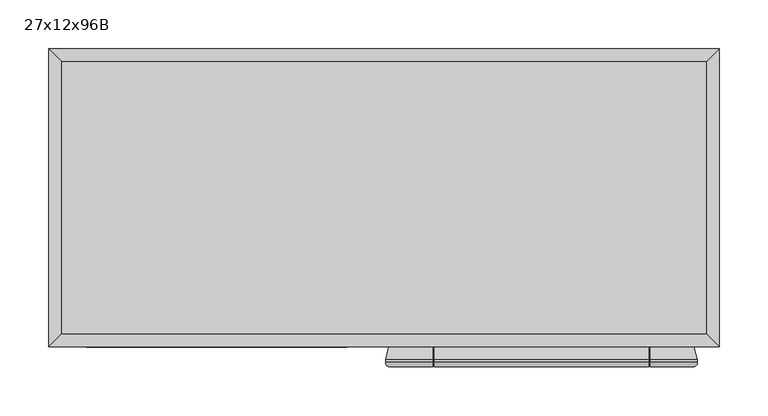
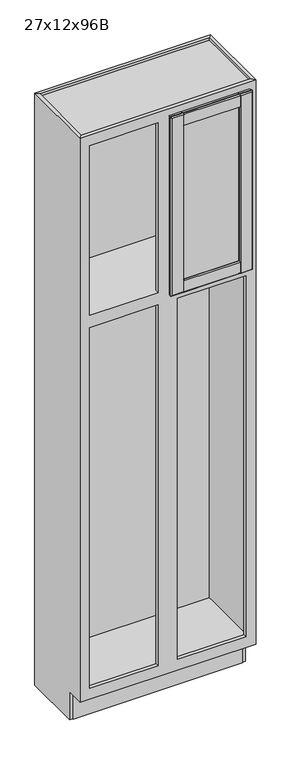
"""IFC4 building model written with IfcOpenShell, lengths in millimetres: furniture geometry, Cabinet-Tall-Merillat-Utility_Double-Marlin : 27x12x96B."""

from ifc_helpers import new_model, si_unit, frame, origin, origin_with_axes, place, context, project, spatial, polyline, circle_curve, ellipse_curve, outline, extrude, faceted_brep, source, transform, mapped, element, save
from ifc_brep_helpers import plane_surface, cylinder_surface, advanced_brep


def furniture_27x12x96b_0ef1cbea(model_context):
    return source(origin(), model_context, "Body", "SolidModel", [
        advanced_brep(
        [(314.6646592, -320.6496, 2413.0), (311.5681667, -325.12, 2409.9035075), (311.5681667, -325.12, 1679.4964925), (314.6646592, -320.6496, 1676.4), (314.6646592, -317.881, 1676.4), (314.6646592, -317.881, 2413.0), (311.1594592, -304.8, 1679.9052), (311.1594592, -304.8, 2409.4948), (266.4634964, -304.8, 2364.7988372), (266.4634964, -304.8, 1724.6011628), (266.0933647, -305.59375, 1724.9712945), (264.0122057, -310.05681, 1727.0524535), (264.0122057, -310.05681, 2362.3475465), (266.0933647, -305.59375, 2364.4287055), (265.4119751, -312.2969093, 1725.652684), (265.4119751, -312.2969093, 2363.747316), (279.7396592, -312.547, 1711.325), (279.7396592, -312.547, 2378.075), (279.7396592, -317.373, 1711.325), (279.7396592, -317.373, 2378.075), (265.4119751, -317.6230907, 1725.652684), (265.4119751, -317.6230907, 2363.747316), (264.0122057, -319.86319, 1727.0524535), (264.0122057, -319.86319, 2362.3475465), (266.0933647, -324.32625, 1724.9712945), (266.460629, -325.1138508, 1724.6040302), (266.4634964, -325.12, 2364.7988372), (266.0933647, -324.32625, 2364.4287055), (266.460629, -325.12, 1679.4964925), (266.460629, -320.6496, 1676.4), (-1.3263483, -325.12, 1679.4964925), (-4.4228408, -320.6496, 1676.4), (43.7413778, -320.6496, 1676.4), (43.7413778, -325.12, 1679.4964925), (264.873129, -320.6496, 1676.4), (264.873129, -325.12, 1679.4964925), (45.3288778, -325.12, 1679.4964925), (45.3288778, -320.6496, 1676.4), (266.460629, -317.881, 1676.4), (-4.4228408, -317.881, 1676.4), (43.7413778, -317.881, 1676.4), (264.873129, -317.881, 1676.4), (45.3288778, -317.881, 1676.4), (266.460629, -304.8, 1679.9052), (-0.9176408, -304.8, 1679.9052), (43.7413778, -304.8, 1679.9052), (264.873129, -304.8, 1679.9052), (45.3288778, -304.8, 1679.9052), (46.2296127, -310.05681, 1727.0524535), (264.873129, -305.59375, 1724.9712945), (264.873129, -304.8, 1724.6011628), (45.3288778, -304.8, 1724.6011628), (45.3288778, -305.59375, 1724.9712945), (44.1484536, -305.59375, 1724.9712945), (44.8298432, -312.2969093, 1725.652684), (30.5021592, -312.547, 1711.325), (30.5021592, -317.373, 1711.325), (44.8298432, -317.6230907, 1725.652684), (46.2296127, -319.86319, 1727.0524535), (44.1484536, -324.32625, 1724.9712945), (45.3288778, -324.32625, 1724.9712945), (45.3288778, -325.12, 1724.6011628), (264.873129, -325.12, 1724.6011628), (264.873129, -324.32625, 1724.9712945), (-1.3263483, -325.12, 2409.9035075), (-4.4228408, -320.6496, 2413.0), (-4.4228408, -317.881, 2413.0), (-0.9176408, -304.8, 2409.4948), (43.7783219, -304.8, 1724.6011628), (43.7783219, -304.8, 2364.7988372), (44.1484536, -305.59375, 2364.4287055), (46.2296127, -310.05681, 2362.3475465), (44.8298432, -312.2969093, 2363.747316), (30.5021592, -312.547, 2378.075), (30.5021592, -317.373, 2378.075), (44.8298432, -317.6230907, 2363.747316), (46.2296127, -319.86319, 2362.3475465), (44.1484536, -324.32625, 2364.4287055), (43.7783219, -325.12, 2364.7988372), (43.7783219, -325.12, 1724.6011628), (43.7413778, -325.12, 2409.9035075), (43.7413778, -320.6496, 2413.0), (266.460629, -320.6496, 2413.0), (266.460629, -325.12, 2409.9035075), (45.3288778, -320.6496, 2413.0), (45.3288778, -325.12, 2409.9035075), (264.873129, -325.12, 2409.9035075), (264.873129, -320.6496, 2413.0), (43.7413778, -317.881, 2413.0), (266.460629, -317.881, 2413.0), (45.3288778, -317.881, 2413.0), (264.873129, -317.881, 2413.0), (43.7413778, -304.8, 2409.4948), (266.460629, -304.8, 2409.4948), (45.3288778, -304.8, 2409.4948), (264.873129, -304.8, 2409.4948), (45.3288778, -304.8, 2364.7988372), (264.873129, -304.8, 2364.7988372), (45.3288778, -305.59375, 2364.4287055), (264.873129, -305.59375, 2364.4287055), (264.873129, -324.32625, 2364.4287055), (264.873129, -325.12, 2364.7988372), (45.3288778, -325.12, 2364.7988372), (45.3288778, -324.32625, 2364.4287055), (45.3288778, -305.59375, 2408.8857412), (45.3288778, -317.9855037, 2412.20625), (45.3288778, -320.6496, 2412.20625), (45.3288778, -324.32625, 2409.7526052), (43.7413778, -324.32625, 2364.4287055), (43.7413778, -324.32625, 2409.7526052), (43.7413778, -320.6496, 2412.20625), (43.7413778, -317.9855037, 2412.20625), (43.7413778, -305.59375, 2408.8857412), (43.7413778, -305.59375, 2364.4287055), (266.460629, -305.59375, 2364.4287055), (266.460629, -305.59375, 2408.8857412), (266.460629, -317.9855037, 2412.20625), (266.460629, -320.6496, 2412.20625), (266.460629, -324.32625, 2409.7526052), (266.460629, -324.32625, 2364.4287055), (264.873129, -324.32625, 2409.7526052), (264.873129, -320.6496, 2412.20625), (264.873129, -317.9855037, 2412.20625), (264.873129, -305.59375, 2408.8857412), (266.460629, -324.32625, 1724.9712945), (266.460629, -324.32625, 1679.6473948), (266.460629, -320.6496, 1677.19375), (266.460629, -317.9855037, 1677.19375), (266.460629, -305.59375, 1680.5142588), (266.460629, -305.59375, 1724.9712945), (264.873129, -305.59375, 1680.5142588), (264.873129, -317.9855037, 1677.19375), (264.873129, -320.6496, 1677.19375), (264.873129, -324.32625, 1679.6473948), (45.3288778, -324.32625, 1679.6473948), (45.3288778, -320.6496, 1677.19375), (45.3288778, -317.9855037, 1677.19375), (45.3288778, -305.59375, 1680.5142588), (43.7413778, -324.32625, 1724.9712945), (43.7413778, -305.59375, 1724.9712945), (43.7413778, -305.59375, 1680.5142588), (43.7413778, -317.9855037, 1677.19375), (43.7413778, -320.6496, 1677.19375), (43.7413778, -324.32625, 1679.6473948)],
        [
            (0, 1, ellipse_curve(frame((309.8894592, -320.6496, 2408.2248), z_axis=(0.7071067811865475, 0.0, -0.7071067811865475), x_axis=(0.7071067811865474, 0.0, 0.7071067811865476)), 6.7531526, 4.7752)),
            (1, 2),
            (2, 3, ellipse_curve(frame((309.8894592, -320.6496, 1681.1752), z_axis=(0.7071067811865475, 0.0, 0.7071067811865475), x_axis=(-0.7071067811865474, 0.0, 0.7071067811865476)), 6.7531526, 4.7752)),
            (3, 0),
            (3, 4),
            (4, 5),
            (5, 0),
            (4, 6),
            (6, 7),
            (7, 5),
            (8, 9),
            (9, 10),
            (10, 11),
            (11, 12),
            (12, 13),
            (13, 8),
            (11, 14, ellipse_curve(frame((265.4394592, -310.7223492, 1725.6252), z_axis=(0.7071067811865475, 0.0, 0.7071067811865475), x_axis=(-0.7071067811865474, 0.0, 0.7071067811865476)), 2.2271035, 1.5748)),
            (14, 15),
            (15, 12, ellipse_curve(frame((265.4394592, -310.7223492, 2363.7748), z_axis=(0.7071067811865475, 0.0, -0.7071067811865475), x_axis=(0.7071067811865474, 0.0, 0.7071067811865476)), 2.2271035, 1.5748)),
            (14, 16),
            (16, 17),
            (17, 15),
            (16, 18),
            (18, 19),
            (19, 17),
            (18, 20),
            (20, 21),
            (21, 19),
            (20, 22, ellipse_curve(frame((265.4394592, -319.1976508, 1725.6252), z_axis=(0.7071067811865475, 0.0, 0.7071067811865475), x_axis=(-0.7071067811865474, 0.0, 0.7071067811865476)), 2.2271035, 1.5748)),
            (22, 23),
            (23, 21, ellipse_curve(frame((265.4394592, -319.1976508, 2363.7748), z_axis=(0.7071067811865475, 0.0, -0.7071067811865475), x_axis=(0.7071067811865474, 0.0, 0.7071067811865476)), 2.2271035, 1.5748)),
            (22, 24),
            (24, 25),
            (25, 26),
            (26, 27),
            (27, 23),
            (2, 28),
            (28, 29, circle_curve(frame((266.460629, -320.6496, 1681.1752), z_axis=(1.0, 0.0, 0.0), x_axis=(0.0, 1.0, 0.0)), 4.7752)),
            (29, 3),
            (30, 31, ellipse_curve(frame((0.3523592, -320.6496, 1681.1752), z_axis=(0.7071067811865475, 0.0, -0.7071067811865475), x_axis=(0.7071067811865476, 0.0, 0.7071067811865474)), 6.7531526, 4.7752)),
            (31, 32),
            (32, 33, circle_curve(frame((43.7413778, -320.6496, 1681.1752), z_axis=(-1.0, 0.0, 0.0), x_axis=(0.0, 1.0, 0.0)), 4.7752)),
            (33, 30),
            (34, 35, circle_curve(frame((264.873129, -320.6496, 1681.1752), z_axis=(-1.0, 0.0, 0.0), x_axis=(0.0, 1.0, 0.0)), 4.7752)),
            (35, 36),
            (36, 37, circle_curve(frame((45.3288778, -320.6496, 1681.1752), z_axis=(1.0, 0.0, 0.0), x_axis=(0.0, 1.0, 0.0)), 4.7752)),
            (37, 34),
            (29, 38),
            (38, 4),
            (31, 39),
            (39, 40),
            (40, 32),
            (41, 34),
            (37, 42),
            (42, 41),
            (38, 43),
            (43, 6),
            (39, 44),
            (44, 45),
            (45, 40),
            (46, 41),
            (42, 47),
            (47, 46),
            (48, 11),
            (10, 49),
            (49, 50),
            (50, 51),
            (51, 52),
            (52, 53),
            (53, 48),
            (48, 54, ellipse_curve(frame((44.8023592, -310.7223492, 1725.6252), z_axis=(0.7071067811865475, 0.0, -0.7071067811865475), x_axis=(0.7071067811865476, 0.0, 0.7071067811865474)), 2.2271035, 1.5748)),
            (54, 14),
            (54, 55),
            (55, 16),
            (55, 56),
            (56, 18),
            (56, 57),
            (57, 20),
            (57, 58, ellipse_curve(frame((44.8023592, -319.1976508, 1725.6252), z_axis=(0.7071067811865475, 0.0, -0.7071067811865475), x_axis=(0.7071067811865476, 0.0, 0.7071067811865474)), 2.2271035, 1.5748)),
            (58, 22),
            (58, 59),
            (59, 60),
            (60, 61),
            (61, 62),
            (62, 63),
            (63, 24),
            (30, 64),
            (64, 65, ellipse_curve(frame((0.3523592, -320.6496, 2408.2248), z_axis=(-0.7071067811865475, 0.0, -0.7071067811865475), x_axis=(0.7071067811865474, 0.0, -0.7071067811865476)), 6.7531526, 4.7752)),
            (65, 31),
            (65, 66),
            (66, 39),
            (66, 67),
            (67, 44),
            (68, 69),
            (69, 70),
            (70, 71),
            (71, 48),
            (53, 68),
            (71, 72, ellipse_curve(frame((44.8023592, -310.7223492, 2363.7748), z_axis=(-0.7071067811865475, 0.0, -0.7071067811865475), x_axis=(0.7071067811865474, 0.0, -0.7071067811865476)), 2.2271035, 1.5748)),
            (72, 54),
            (72, 73),
            (73, 55),
            (73, 74),
            (74, 56),
            (74, 75),
            (75, 57),
            (75, 76, ellipse_curve(frame((44.8023592, -319.1976508, 2363.7748), z_axis=(-0.7071067811865475, 0.0, -0.7071067811865475), x_axis=(0.7071067811865474, 0.0, -0.7071067811865476)), 2.2271035, 1.5748)),
            (76, 58),
            (76, 77),
            (77, 78),
            (78, 79),
            (79, 59),
            (64, 80),
            (80, 81, circle_curve(frame((43.7413778, -320.6496, 2408.2248), z_axis=(-1.0, 0.0, 0.0), x_axis=(0.0, 1.0, 0.0)), 4.7752)),
            (81, 65),
            (0, 82),
            (82, 83, circle_curve(frame((266.460629, -320.6496, 2408.2248), z_axis=(1.0, 0.0, 0.0), x_axis=(0.0, 1.0, 0.0)), 4.7752)),
            (83, 1),
            (84, 85, circle_curve(frame((45.3288778, -320.6496, 2408.2248), z_axis=(1.0, 0.0, 0.0), x_axis=(0.0, 1.0, 0.0)), 4.7752)),
            (85, 86),
            (86, 87, circle_curve(frame((264.873129, -320.6496, 2408.2248), z_axis=(-1.0, 0.0, 0.0), x_axis=(0.0, 1.0, 0.0)), 4.7752)),
            (87, 84),
            (81, 88),
            (88, 66),
            (5, 89),
            (89, 82),
            (90, 84),
            (87, 91),
            (91, 90),
            (88, 92),
            (92, 67),
            (7, 93),
            (93, 89),
            (94, 90),
            (91, 95),
            (95, 94),
            (43, 9),
            (8, 93),
            (92, 69),
            (68, 45),
            (96, 94),
            (95, 97),
            (97, 96),
            (50, 46),
            (47, 51),
            (12, 71),
            (70, 98),
            (98, 96),
            (97, 99),
            (99, 13),
            (15, 72),
            (17, 73),
            (19, 74),
            (21, 75),
            (23, 76),
            (27, 100),
            (100, 101),
            (101, 102),
            (102, 103),
            (103, 77),
            (83, 26),
            (25, 28),
            (33, 79),
            (78, 80),
            (85, 102),
            (101, 86),
            (35, 62),
            (61, 36),
            (98, 104),
            (104, 105),
            (105, 106),
            (106, 107, circle_curve(frame((45.3288778, -320.6496, 2408.2248), z_axis=(1.0, 0.0, 0.0), x_axis=(0.0, 0.0, 1.0)), 3.98145)),
            (107, 103),
            (78, 108),
            (108, 109),
            (109, 110, circle_curve(frame((43.7413778, -320.6496, 2408.2248), z_axis=(-1.0, 0.0, 0.0), x_axis=(0.0, 0.0, 1.0)), 3.98145)),
            (110, 111),
            (111, 112),
            (112, 113),
            (113, 69),
            (77, 108),
            (107, 109),
            (106, 110),
            (105, 111),
            (104, 112),
            (70, 113),
            (8, 114),
            (114, 115),
            (115, 116),
            (116, 117),
            (117, 118, circle_curve(frame((266.460629, -320.6496, 2408.2248), z_axis=(1.0, 0.0, 0.0), x_axis=(0.0, 0.0, 1.0)), 3.98145)),
            (118, 119),
            (119, 26),
            (100, 120),
            (120, 121, circle_curve(frame((264.873129, -320.6496, 2408.2248), z_axis=(-1.0, 0.0, 0.0), x_axis=(0.0, 0.0, 1.0)), 3.98145)),
            (121, 122),
            (122, 123),
            (123, 99),
            (119, 27),
            (118, 120),
            (117, 121),
            (116, 122),
            (115, 123),
            (114, 13),
            (25, 124),
            (124, 125),
            (125, 126, circle_curve(frame((266.460629, -320.6496, 1681.1752), z_axis=(1.0, 0.0, 0.0), x_axis=(0.0, 0.0, 1.0)), 3.98145)),
            (126, 127),
            (127, 128),
            (128, 129),
            (129, 9),
            (49, 130),
            (130, 131),
            (131, 132),
            (132, 133, circle_curve(frame((264.873129, -320.6496, 1681.1752), z_axis=(-1.0, 0.0, 0.0), x_axis=(0.0, 0.0, 1.0)), 3.98145)),
            (133, 63),
            (129, 10),
            (128, 130),
            (127, 131),
            (126, 132),
            (125, 133),
            (124, 24),
            (60, 134),
            (134, 135, circle_curve(frame((45.3288778, -320.6496, 1681.1752), z_axis=(1.0, 0.0, 0.0), x_axis=(0.0, 0.0, 1.0)), 3.98145)),
            (135, 136),
            (136, 137),
            (137, 52),
            (138, 79),
            (68, 139),
            (139, 140),
            (140, 141),
            (141, 142),
            (142, 143, circle_curve(frame((43.7413778, -320.6496, 1681.1752), z_axis=(-1.0, 0.0, 0.0), x_axis=(0.0, 0.0, 1.0)), 3.98145)),
            (143, 138),
            (138, 59),
            (53, 139),
            (137, 140),
            (136, 141),
            (135, 142),
            (134, 143),
        ],
        [
            cylinder_surface(frame((309.8894592, -320.6496, 2413.0), z_axis=(0.0, 0.0, 1.0), x_axis=(0.0, 1.0, 0.0)), 4.7752),
            plane_surface(frame((314.6646592, -320.6496, 2413.0), z_axis=(1.0, 0.0, 0.0), x_axis=(0.0, 0.0, -1.0))),
            plane_surface(frame((314.6646592, -317.881, 2413.0), z_axis=(0.9659229350723619, 0.25882983502910506, 0.0), x_axis=(0.0, 0.0, -1.0))),
            plane_surface(frame((266.4634964, -304.8, 2364.7988372), z_axis=(-0.9063077870366099, 0.4226182617407856, 0.0), x_axis=(0.0, 0.0, -1.0))),
            cylinder_surface(frame((265.4394592, -310.7223492, 2413.0), z_axis=(0.0, 0.0, 1.0000000000000002), x_axis=(-0.01745240643729364, -0.9998476951563912, 0.0)), 1.5748),
            plane_surface(frame((265.4119751, -312.2969093, 2363.747316), z_axis=(-0.017452406437322144, -0.9998476951563906, 0.0), x_axis=(0.0, 0.0, -1.0))),
            plane_surface(frame((279.7396592, -312.547, 2378.075), z_axis=(-1.0, 0.0, 0.0), x_axis=(0.0, 0.0, -1.0))),
            plane_surface(frame((279.7396592, -317.373, 2378.075), z_axis=(-0.01745240643727848, 0.9998476951563914, 0.0), x_axis=(0.0, 0.0, -1.0))),
            cylinder_surface(frame((265.4394592, -319.1976508, 2413.0), z_axis=(0.0, 0.0, 1.0000000000000002), x_axis=(-0.9063077870367326, -0.42261826174052236, 0.0)), 1.5748),
            plane_surface(frame((264.0122057, -319.86319, 2362.3475465), z_axis=(-0.9063077870366333, -0.4226182617407352, 0.0), x_axis=(0.0, 0.0, -1.0))),
            cylinder_surface(frame((314.6646592, -320.6496, 1681.1752), z_axis=(1.0, 0.0, 0.0), x_axis=(0.0, 1.0, 0.0)), 4.7752),
            plane_surface(frame((314.6646592, -320.6496, 1676.4), z_axis=(0.0, 0.0, -1.0), x_axis=(-1.0, 0.0, 0.0))),
            plane_surface(frame((314.6646592, -317.881, 1676.4), z_axis=(0.0, 0.25882983502910506, -0.9659229350723619), x_axis=(-1.0, 0.0, 0.0))),
            plane_surface(frame((266.4634964, -304.8, 1724.6011628), z_axis=(0.0, 0.4226182617407856, 0.9063077870366099), x_axis=(-1.0, 0.0, 0.0))),
            cylinder_surface(frame((314.6646592, -310.7223492, 1725.6252), z_axis=(1.0000000000000002, 0.0, 0.0), x_axis=(0.0, -0.9998476951563912, 0.01745240643729364)), 1.5748),
            plane_surface(frame((265.4119751, -312.2969093, 1725.652684), z_axis=(0.0, -0.9998476951563906, 0.017452406437322144), x_axis=(-1.0, 0.0, 0.0))),
            plane_surface(frame((279.7396592, -312.547, 1711.325), z_axis=(0.0, 0.0, 1.0), x_axis=(-1.0, 0.0, 0.0))),
            plane_surface(frame((279.7396592, -317.373, 1711.325), z_axis=(0.0, 0.9998476951563914, 0.01745240643727848), x_axis=(-1.0, 0.0, 0.0))),
            cylinder_surface(frame((314.6646592, -319.1976508, 1725.6252), z_axis=(1.0000000000000002, 0.0, 0.0), x_axis=(0.0, -0.42261826174052236, 0.9063077870367326)), 1.5748),
            plane_surface(frame((264.0122057, -319.86319, 1727.0524535), z_axis=(0.0, -0.4226182617407352, 0.9063077870366333), x_axis=(-1.0, 0.0, 0.0))),
            cylinder_surface(frame((0.3523592, -320.6496, 1676.4), z_axis=(0.0, 0.0, -1.0), x_axis=(0.0, 1.0, 0.0)), 4.7752),
            plane_surface(frame((-4.4228408, -320.6496, 1676.4), z_axis=(-1.0, 0.0, 0.0), x_axis=(0.0, 0.0, 1.0))),
            plane_surface(frame((-4.4228408, -317.881, 1676.4), z_axis=(-0.9659229350723619, 0.25882983502910506, 0.0), x_axis=(0.0, 0.0, 1.0))),
            plane_surface(frame((43.7783219, -304.8, 1724.6011628), z_axis=(0.9063077870366099, 0.4226182617407856, 0.0), x_axis=(0.0, 0.0, 1.0))),
            cylinder_surface(frame((44.8023592, -310.7223492, 1676.4), z_axis=(0.0, 0.0, -1.0000000000000002), x_axis=(0.01745240643729364, -0.9998476951563912, 0.0)), 1.5748),
            plane_surface(frame((44.8298432, -312.2969093, 1725.652684), z_axis=(0.017452406437322144, -0.9998476951563906, 0.0), x_axis=(0.0, 0.0, 1.0))),
            plane_surface(frame((30.5021592, -312.547, 1711.325), z_axis=(1.0, 0.0, 0.0), x_axis=(0.0, 0.0, 1.0))),
            plane_surface(frame((30.5021592, -317.373, 1711.325), z_axis=(0.01745240643727848, 0.9998476951563914, 0.0), x_axis=(0.0, 0.0, 1.0))),
            cylinder_surface(frame((44.8023592, -319.1976508, 1676.4), z_axis=(0.0, 0.0, -1.0000000000000002), x_axis=(0.9063077870367326, -0.42261826174052236, 0.0)), 1.5748),
            plane_surface(frame((46.2296127, -319.86319, 1727.0524535), z_axis=(0.9063077870366333, -0.4226182617407352, 0.0), x_axis=(0.0, 0.0, 1.0))),
            cylinder_surface(frame((-4.4228408, -320.6496, 2408.2248), z_axis=(-1.0, 0.0, 0.0), x_axis=(0.0, 1.0, 0.0)), 4.7752),
            plane_surface(frame((-4.4228408, -320.6496, 2413.0), z_axis=(0.0, 0.0, 1.0), x_axis=(1.0, 0.0, 0.0))),
            plane_surface(frame((-4.4228408, -317.881, 2413.0), z_axis=(0.0, 0.25882983502910506, 0.9659229350723619), x_axis=(1.0, 0.0, 0.0))),
            plane_surface(frame((-0.9176408, -304.8, 2409.4948), z_axis=(0.0, 1.0, 0.0), x_axis=(1.0, 0.0, 0.0))),
            plane_surface(frame((43.7783219, -304.8, 2364.7988372), z_axis=(0.0, 0.4226182617407856, -0.9063077870366099), x_axis=(1.0, 0.0, 0.0))),
            cylinder_surface(frame((-4.4228408, -310.7223492, 2363.7748), z_axis=(-1.0000000000000002, 0.0, 0.0), x_axis=(0.0, -0.9998476951563912, -0.01745240643729364)), 1.5748),
            plane_surface(frame((44.8298432, -312.2969093, 2363.747316), z_axis=(0.0, -0.9998476951563906, -0.017452406437322144), x_axis=(1.0, 0.0, 0.0))),
            plane_surface(frame((30.5021592, -312.547, 2378.075), z_axis=(0.0, 0.0, -1.0), x_axis=(1.0, 0.0, 0.0))),
            plane_surface(frame((30.5021592, -317.373, 2378.075), z_axis=(0.0, 0.9998476951563914, -0.01745240643727848), x_axis=(1.0, 0.0, 0.0))),
            cylinder_surface(frame((-4.4228408, -319.1976508, 2363.7748), z_axis=(-1.0000000000000002, 0.0, 0.0), x_axis=(0.0, -0.42261826174052236, -0.9063077870367326)), 1.5748),
            plane_surface(frame((46.2296127, -319.86319, 2362.3475465), z_axis=(0.0, -0.4226182617407352, -0.9063077870366333), x_axis=(1.0, 0.0, 0.0))),
            plane_surface(frame((43.7783219, -325.12, 2364.7988372), z_axis=(0.0, -1.0, 0.0), x_axis=(1.0, 0.0, 0.0))),
            plane_surface(frame((45.3288778, -325.12, 2364.7988372), z_axis=(-1.0000000000000002, 0.0, 0.0), x_axis=(0.0, 0.9063077870366255, -0.4226182617407521))),
            plane_surface(frame((43.7413778, -325.12, 2364.7988372), z_axis=(1.0000000000000002, 0.0, 0.0), x_axis=(0.0, -0.9063077870366255, 0.4226182617407521))),
            plane_surface(frame((45.3288778, -325.12, 2364.7988372), z_axis=(0.0, 0.4226182617407521, 0.9063077870366255), x_axis=(-1.0, 0.0, 0.0))),
            plane_surface(frame((45.3288778, -324.32625, 2364.4287055), z_axis=(0.0, -1.0, 0.0), x_axis=(-1.0, 0.0, 0.0))),
            cylinder_surface(frame((43.7413778, -320.6496, 2408.2248), z_axis=(-1.0, 0.0, 0.0), x_axis=(0.0, 0.0, 1.0)), 3.98145),
            plane_surface(frame((45.3288778, -320.6496, 2412.20625), z_axis=(0.0, 0.0, 1.0), x_axis=(-1.0, 0.0, 0.0))),
            plane_surface(frame((45.3288778, -317.9855037, 2412.20625), z_axis=(0.0, 0.25882983502916707, 0.9659229350723454), x_axis=(-1.0, 0.0, 0.0))),
            plane_surface(frame((45.3288778, -305.59375, 2408.8857412), z_axis=(0.0, 1.0, 0.0), x_axis=(-1.0, 0.0, 0.0))),
            plane_surface(frame((45.3288778, -305.59375, 2364.4287055), z_axis=(0.0, -0.42261826174074746, 0.9063077870366276), x_axis=(-1.0, 0.0, 0.0))),
            plane_surface(frame((266.460629, -325.12, 2364.7988372), z_axis=(-1.0, 0.0, 0.0), x_axis=(0.0, 0.9063077870366341, -0.4226182617407336))),
            plane_surface(frame((264.873129, -325.12, 2364.7988372), z_axis=(1.0, 0.0, 0.0), x_axis=(0.0, -0.9063077870366341, 0.4226182617407336))),
            plane_surface(frame((266.460629, -325.12, 2364.7988372), z_axis=(0.0, 0.4226182617407336, 0.9063077870366341), x_axis=(-1.0, 0.0, 0.0))),
            plane_surface(frame((266.460629, -324.32625, 2364.4287055), z_axis=(0.0, -1.0, 0.0), x_axis=(-1.0, 0.0, 0.0))),
            cylinder_surface(frame((264.873129, -320.6496, 2408.2248), z_axis=(-1.0, 0.0, 0.0), x_axis=(0.0, 0.0, 1.0)), 3.98145),
            plane_surface(frame((266.460629, -320.6496, 2412.20625), z_axis=(0.0, 0.0, 1.0), x_axis=(-1.0, 0.0, 0.0))),
            plane_surface(frame((266.460629, -317.9855037, 2412.20625), z_axis=(0.0, 0.25882983502916396, 0.9659229350723462), x_axis=(-1.0, 0.0, 0.0))),
            plane_surface(frame((266.460629, -305.59375, 2408.8857412), z_axis=(0.0, 1.0, 0.0), x_axis=(-1.0, 0.0, 0.0))),
            plane_surface(frame((266.460629, -305.59375, 2364.4287055), z_axis=(0.0, -0.4226182617407683, 0.9063077870366179), x_axis=(-1.0, 0.0, 0.0))),
            plane_surface(frame((266.460629, -320.6496, 1685.9504), z_axis=(-1.0, 0.0, 0.0), x_axis=(0.0, -1.0, 0.0))),
            plane_surface(frame((264.873129, -320.6496, 1685.9504), z_axis=(1.0, 0.0, 0.0), x_axis=(0.0, 1.0, 0.0))),
            plane_surface(frame((266.460629, -304.8, 1724.6011628), z_axis=(0.0, -0.42261826174076006, -0.9063077870366217), x_axis=(-1.0, 0.0, 0.0))),
            plane_surface(frame((266.460629, -305.59375, 1724.9712945), z_axis=(0.0, 1.0, 0.0), x_axis=(-1.0, 0.0, 0.0))),
            plane_surface(frame((266.460629, -305.59375, 1680.5142588), z_axis=(0.0, 0.2588298350294376, -0.9659229350722728), x_axis=(-1.0, 0.0, 0.0))),
            plane_surface(frame((266.460629, -317.9855037, 1677.19375), z_axis=(0.0, 0.0, -1.0), x_axis=(-1.0, 0.0, 0.0))),
            cylinder_surface(frame((264.873129, -320.6496, 1681.1752), z_axis=(-1.0, 0.0, 0.0), x_axis=(0.0, 0.0, 1.0)), 3.98145),
            plane_surface(frame((266.460629, -324.32625, 1679.6473948), z_axis=(0.0, -1.0, 0.0), x_axis=(-1.0, 0.0, 0.0))),
            plane_surface(frame((266.460629, -324.32625, 1724.9712945), z_axis=(0.0, 0.42261826174073647, -0.9063077870366327), x_axis=(-1.0, 0.0, 0.0))),
            plane_surface(frame((45.3288778, -324.32625, 1724.9712945), z_axis=(-1.0, 0.0, 0.0), x_axis=(0.0, -0.9063077870366145, -0.42261826174077555))),
            plane_surface(frame((43.7413778, -324.32625, 1724.9712945), z_axis=(1.0, 0.0, 0.0), x_axis=(0.0, 0.9063077870366145, 0.42261826174077555))),
            plane_surface(frame((45.3288778, -324.32625, 1724.9712945), z_axis=(0.0, 0.42261826174077555, -0.9063077870366145), x_axis=(-1.0, 0.0, 0.0))),
            plane_surface(frame((45.3288778, -304.8, 1724.6011628), z_axis=(0.0, -0.4226182617407416, -0.9063077870366304), x_axis=(-1.0, 0.0, 0.0))),
            plane_surface(frame((45.3288778, -305.59375, 1724.9712945), z_axis=(0.0, 1.0, 0.0), x_axis=(-1.0, 0.0, 0.0))),
            plane_surface(frame((45.3288778, -305.59375, 1680.5142588), z_axis=(0.0, 0.2588298350294381, -0.9659229350722727), x_axis=(-1.0, 0.0, 0.0))),
            plane_surface(frame((45.3288778, -317.9855037, 1677.19375), z_axis=(0.0, 0.0, -1.0), x_axis=(-1.0, 0.0, 0.0))),
            cylinder_surface(frame((43.7413778, -320.6496, 1681.1752), z_axis=(-1.0, 0.0, 0.0), x_axis=(0.0, 0.0, 1.0)), 3.98145),
            plane_surface(frame((45.3288778, -324.32625, 1679.6473948), z_axis=(0.0, -1.0, 0.0), x_axis=(-1.0, 0.0, 0.0))),
        ],
        [
            (0, [[1, 2, 3, 4]]),
            (1, [[-4, 5, 6, 7]]),
            (2, [[-6, 8, 9, 10]]),
            (3, [[11, 12, 13, 14, 15, 16]]),
            (4, [[-14, 17, 18, 19]]),
            (5, [[-18, 20, 21, 22]]),
            (6, [[-21, 23, 24, 25]]),
            (7, [[-24, 26, 27, 28]]),
            (8, [[-27, 29, 30, 31]]),
            (9, [[-30, 32, 33, 34, 35, 36]]),
            (10, [[-3, 37, 38, 39]]),
            (10, [[40, 41, 42, 43]]),
            (10, [[44, 45, 46, 47]]),
            (11, [[-5, -39, 48, 49]]),
            (11, [[50, 51, 52, -41]]),
            (11, [[53, -47, 54, 55]]),
            (12, [[-8, -49, 56, 57]]),
            (12, [[58, 59, 60, -51]]),
            (12, [[61, -55, 62, 63]]),
            (13, [[64, -13, 65, 66, 67, 68, 69, 70]]),
            (14, [[-17, -64, 71, 72]]),
            (15, [[-20, -72, 73, 74]]),
            (16, [[-23, -74, 75, 76]]),
            (17, [[-26, -76, 77, 78]]),
            (18, [[-29, -78, 79, 80]]),
            (19, [[-80, 81, 82, 83, 84, 85, 86, -32]]),
            (20, [[-40, 87, 88, 89]]),
            (21, [[-50, -89, 90, 91]]),
            (22, [[-58, -91, 92, 93]]),
            (23, [[94, 95, 96, 97, -70, 98]]),
            (24, [[-71, -97, 99, 100]]),
            (25, [[-73, -100, 101, 102]]),
            (26, [[-75, -102, 103, 104]]),
            (27, [[-77, -104, 105, 106]]),
            (28, [[-79, -106, 107, 108]]),
            (29, [[-108, 109, 110, 111, 112, -81]]),
            (30, [[-88, 113, 114, 115]]),
            (30, [[-1, 116, 117, 118]]),
            (30, [[119, 120, 121, 122]]),
            (31, [[-90, -115, 123, 124]]),
            (31, [[-7, 125, 126, -116]]),
            (31, [[127, -122, 128, 129]]),
            (32, [[-92, -124, 130, 131]]),
            (32, [[-10, 132, 133, -125]]),
            (32, [[134, -129, 135, 136]]),
            (33, [[-9, -57, 137, -11, 138, -132]]),
            (33, [[-93, -131, 139, -94, 140, -59]]),
            (33, [[141, -136, 142, 143]]),
            (33, [[144, -63, 145, -67]]),
            (34, [[146, -96, 147, 148, -143, 149, 150, -15]]),
            (35, [[-19, 151, -99, -146]]),
            (36, [[-22, 152, -101, -151]]),
            (37, [[-25, 153, -103, -152]]),
            (38, [[-28, 154, -105, -153]]),
            (39, [[-31, 155, -107, -154]]),
            (40, [[-155, -36, 156, 157, 158, 159, 160, -109]]),
            (41, [[-2, -118, 161, -34, 162, -37]]),
            (41, [[-87, -43, 163, -111, 164, -113]]),
            (41, [[165, -158, 166, -120]]),
            (41, [[167, -84, 168, -45]]),
            (42, [[169, 170, 171, 172, 173, -159, -165, -119, -127, -134, -141, -148]]),
            (43, [[174, 175, 176, 177, 178, 179, 180, -139, -130, -123, -114, -164]]),
            (44, [[-174, -110, 181]]),
            (45, [[-173, 182, -175, -181, -160]]),
            (46, [[-172, 183, -176, -182]]),
            (47, [[-171, 184, -177, -183]]),
            (48, [[-170, 185, -178, -184]]),
            (49, [[-169, -147, 186, -179, -185]]),
            (50, [[-180, -186, -95]]),
            (51, [[187, 188, 189, 190, 191, 192, 193, -161, -117, -126, -133, -138]]),
            (52, [[194, 195, 196, 197, 198, -149, -142, -135, -128, -121, -166, -157]]),
            (53, [[-193, 199, -35]]),
            (54, [[-192, 200, -194, -156, -199]]),
            (55, [[-191, 201, -195, -200]]),
            (56, [[-190, 202, -196, -201]]),
            (57, [[-189, 203, -197, -202]]),
            (58, [[-188, 204, -150, -198, -203]]),
            (59, [[-187, -16, -204]]),
            (60, [[205, 206, 207, 208, 209, 210, 211, -137, -56, -48, -38, -162]]),
            (61, [[212, 213, 214, 215, 216, -85, -167, -44, -53, -61, -144, -66]]),
            (62, [[-211, 217, -12]]),
            (63, [[-210, 218, -212, -65, -217]]),
            (64, [[-209, 219, -213, -218]]),
            (65, [[-208, 220, -214, -219]]),
            (66, [[-207, 221, -215, -220]]),
            (67, [[-206, 222, -86, -216, -221]]),
            (68, [[-205, -33, -222]]),
            (69, [[223, 224, 225, 226, 227, -68, -145, -62, -54, -46, -168, -83]]),
            (70, [[228, -163, -42, -52, -60, -140, 229, 230, 231, 232, 233, 234]]),
            (71, [[-228, 235, -112]]),
            (72, [[-229, -98, 236]]),
            (73, [[-227, 237, -230, -236, -69]]),
            (74, [[-226, 238, -231, -237]]),
            (75, [[-225, 239, -232, -238]]),
            (76, [[-224, 240, -233, -239]]),
            (77, [[-223, -82, -235, -234, -240]]),
        ],
    ),
        extrude(outline(polyline([(30.5021592, -317.373), (30.5021592, -312.547), (279.7396592, -312.547), (279.7396592, -317.373), (30.5021592, -317.373)])), frame((0.0, 0.0, 1711.325), z_axis=(0.0, 0.0, 1.0), x_axis=(1.0, 0.0, 0.0)), (0.0, 0.0, 1.0), 666.75),
        extrude(outline(polyline([(324.1896592, -12.7), (324.1896592, -292.1), (-336.2103408, -292.1), (-336.2103408, -12.7), (324.1896592, -12.7)])), frame((0.0, 0.0, 2419.35), z_axis=(0.0, 0.0, 1.0), x_axis=(1.0, 0.0, 0.0)), (0.0, 0.0, 1.0), 9.525),
        extrude(outline(polyline([(324.1896592, -234.15625), (324.1896592, -237.1082435), (-336.2103408, -237.1082435), (-336.2103408, -234.15625), (324.1896592, -234.15625)])), origin_with_axes(), (0.0, 0.0, 1.0), 114.3),
        faceted_brep([(324.1896592, -292.1, 2438.4), (324.1896592, -292.1, 114.3), (-336.2103408, -292.1, 114.3), (-336.2103408, -292.1, 2438.4), (-44.1103408, -292.1, 2393.95), (-310.8103408, -292.1, 2393.95), (-310.8103408, -292.1, 1695.45), (-310.8103408, -292.1, 1644.65), (-310.8103408, -292.1, 158.75), (-44.1103408, -292.1, 158.75), (-44.1103408, -292.1, 1644.65), (32.0896592, -292.1, 1644.65), (32.0896592, -292.1, 158.75), (298.5896592, -292.1, 158.75), (298.5896592, -292.1, 1644.65), (298.5896592, -292.1, 1695.45), (298.5896592, -292.1, 2393.95), (32.0896592, -292.1, 2393.95), (32.0896592, -292.1, 1695.45), (-44.1103408, -292.1, 1695.45), (-348.9103408, -304.8, 2438.4), (336.8896592, -304.8, 2438.4), (-348.9103408, -304.8, 114.3), (336.8896592, -304.8, 114.3), (32.0896592, -304.8, 158.75), (32.0896592, -304.8, 1644.65), (298.5896592, -304.8, 1644.65), (298.5896592, -304.8, 158.75), (32.0896592, -304.8, 2393.95), (298.5896592, -304.8, 2393.95), (298.5896592, -304.8, 1695.45), (32.0896592, -304.8, 1695.45), (-310.8103408, -304.8, 158.75), (-310.8103408, -304.8, 1644.65), (-44.1103408, -304.8, 1644.65), (-44.1103408, -304.8, 158.75), (-310.8103408, -304.8, 2393.95), (-44.1103408, -304.8, 2393.95), (-44.1103408, -304.8, 1695.45), (-310.8103408, -304.8, 1695.45), (-336.2103408, -234.15625, 114.3), (-336.2103408, -12.7, 114.3), (-336.2103408, -12.7, 2438.4), (-348.9103408, 0.0, 2438.4), (-348.9103408, 0.0, 0.0), (-348.9103408, -234.15625, 0.0), (-348.9103408, -234.15625, 114.3), (324.1896592, -12.7, 114.3), (324.1896592, -12.7, 2438.4), (298.5896592, -12.7, 1695.45), (298.5896592, -12.7, 1644.65), (-310.8103408, -12.7, 1644.65), (-310.8103408, -12.7, 1695.45), (336.8896592, 0.0, 2438.4), (336.8896592, 0.0, 0.0), (324.1896592, -234.15625, 114.3), (336.8896592, -234.15625, 114.3), (336.8896592, -234.15625, 0.0)], [[[0, 1, 2, 3], [4, 5, 6, 7, 8, 9, 10, 11, 12, 13, 14, 15, 16, 17, 18, 19]], [[0, 3, 20, 21]], [[21, 20, 22, 23], [24, 25, 26, 27], [28, 29, 30, 31], [32, 33, 34, 35], [36, 37, 38, 39]], [[2, 1, 23, 22]], [[3, 2, 40, 41, 42]], [[20, 3, 42, 43]], [[22, 20, 43, 44, 45, 46]], [[2, 22, 46, 40]], [[42, 41, 47, 48], [49, 50, 51, 52]], [[43, 42, 48, 53]], [[43, 53, 54, 44]], [[1, 0, 48, 47, 55]], [[0, 21, 53, 48]], [[21, 23, 56, 57, 54, 53]], [[23, 1, 55, 56]], [[40, 55, 47, 41]], [[54, 57, 45, 44]], [[45, 57, 56, 55, 40, 46]], [[36, 5, 4, 37]], [[16, 29, 28, 17]], [[5, 36, 39, 6]], [[32, 8, 7, 33]], [[8, 32, 35, 9]], [[27, 13, 12, 24]], [[29, 16, 15, 30]], [[13, 27, 26, 14]], [[37, 4, 19, 38]], [[9, 35, 34, 10]], [[17, 28, 31, 18]], [[24, 12, 11, 25]], [[49, 15, 14, 50]], [[15, 49, 52, 6, 39, 38, 19, 18, 31, 30]], [[6, 52, 51, 7]], [[50, 14, 26, 25, 11, 10, 34, 33, 7, 51]]]),
        extrude(outline(polyline([(324.1896592, -12.7), (324.1896592, -292.1), (-336.2103408, -292.1), (-336.2103408, -12.7), (324.1896592, -12.7)])), frame((0.0, 0.0, 114.3), z_axis=(0.0, 0.0, 1.0), x_axis=(1.0, 0.0, 0.0)), (0.0, 0.0, 1.0), 19.05),
    ])


if __name__ == "__main__":
    model = new_model("IFC4")
    model_context = context("Model", 3, world=origin())
    ifc_project = project(units=[si_unit("LENGTHUNIT", "METRE", prefix="MILLI")], contexts=[model_context])
    site = spatial("IfcSite", under=ifc_project)
    building = spatial("IfcBuilding", under=site)
    placement = place(None, origin())
    furniture_27x12x96b_shape = furniture_27x12x96b_0ef1cbea(model_context)
    element("IfcFurniture", 1, ObjectType="Cabinet-Tall-Merillat-Utility_Double-Marlin : 27x12x96B", at=placement, inside=building, context=model_context, shape_type="MappedRepresentation", body=[
        mapped(furniture_27x12x96b_shape, transform((0.0, 0.0, 0.0), x_axis=(1.0, 0.0, 0.0), y_axis=(0.0, 1.0, 0.0), z_axis=(0.0, 0.0, 1.0))),
    ])
    save(model, "model.ifc")

# Revit data of these elements
# Type "Cabinet-Tall-Merillat-Utility_Double-Marlin : 27x12x96B"
#   URL = "http://www.merillat.com/"
#   Toe Kick Note = "Toe Kick Covering is not included. To be purchased Separately. \r\n\r\n Toe Kick Covering is not included. To be purchased Separately."
#   Product Page URL = "http://www.merillat.com/our-products/rooms/kitchen/"
#   Product Line = "Express"
#   Product Group = "Tall Cabinet"
#   Product Documentation Link = "http://merillatbusiness.com/wp-content/uploads/2014/07/Merillat_Classic_Catalog.pdf"
#   Model = "U3096B"
#   Manufacturer = "Merillat"
#   Finish = "Wood"
#   Description = "Tall Utility Cabinet Double"
#   Construction Type = "Tall Cabinet"
#   Cabinet Construction Note = ""
#   Assembly Code = "C1030410"
#   Spacing = 0' - 1"
#   Door Spacing = 0' - 0 1/8"
#   Cabinet Upper Door Height = 2' - 5"
#   Cabinet Door Width = 1' - 0 9/16"
#   Cabinet Door Height = 4' - 11 1/2"
#   Depth = 1' - 0"
#   Height = 8' - 0"
#   Toe Depth = 0' - 2 25/32"
#   Toe Height = 0' - 4 1/2"
#   Width = 2' - 3"
#   COBie.Type = no
#   Partial Overlay Butt = yes
#   Partial Overlay = no
#   Full Overlay Butt = no
#   Full Overlay = no
#   Elevation Swing Line = yes
#   Toe Kick Material = Wood - Merillat - Raw Particle Board
#   Door Drawer Material = Wood - Merillat - Pecan(1)
#   Cabinet Material = Wood - Merillat - Pecan(1)
#   Cabinet Door Style = element 776454
# Element 1 (IfcFurniture, "Cabinet-Tall-Merillat-Utility_Double-Marlin : 27x12x96B")
#   Materials on its faces: "Wood - Merillat - Pecan(1)", "Wood - Merillat - Raw Particle Board"
# Materials
#   "Wood - Merillat - Raw Particle Board": class "Plastic", colour RGB 80 80 80, transparency 0, Description = "Plastic Laminate - Navy", Cost = 0
#   "Wood - Merillat - Pecan(1)": class "Wood", colour RGB 108 67 43, transparency 0, Cost = 0
